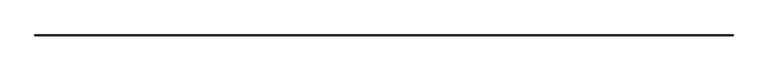
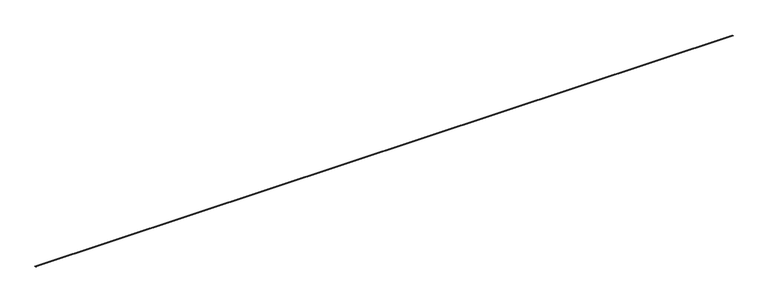
"""IFC4 building model written with IfcOpenShell, lengths in millimetres: proxy geometry, Generic Models 7:Generic Models 1:6:Generic Models 1:6 : Generic Models 7:Generic Models 1:337419:20 : Generic Models 7:Generic Models 1:6:Generic Models 1:6 : Generic Models 7:Generic Models 1:337419:312901."""

from ifc_helpers import new_model, si_unit, frame, origin, place, context, project, spatial, polyline, outline, extrude, source, transform, mapped, element, save


def generic_models_84a8ac5e(model_context):
    return source(origin(), model_context, "Body", "SweptSolid", [
        extrude(outline(polyline([(-579024.8509681, 4.5309106), (-579024.8509681, 24.3756332), (-579021.6759681, 24.3756332), (-579021.6759681, 7.7059106), (-578858.9280519, 7.7059106), (-578858.9280519, 4.5309106), (-579024.8509681, 4.5309106)])), frame((557771.6867239, 0.0, 0.0), z_axis=(1.0, 0.0, 0.0), x_axis=(0.0, 1.0, 0.0)), (0.0, 0.0, 1.0), 109559.725),
    ])


if __name__ == "__main__":
    model = new_model("IFC4")
    model_context = context("Model", 3, world=origin())
    ifc_project = project(units=[si_unit("LENGTHUNIT", "METRE", prefix="MILLI")], contexts=[model_context])
    site = spatial("IfcSite", under=ifc_project)
    building = spatial("IfcBuilding", under=site)
    placement = place(None, origin())
    generic_models_shape = generic_models_84a8ac5e(model_context)
    element("IfcBuildingElementProxy", 1, Name="Generic Models 7:Generic Models 1:6:Generic Models 1:6 : Generic Models 7:Generic Models 1:337419:20 : Generic Models 7:Generic Models 1:6:Generic Models 1:6 : Generic Models 7:Generic Models 1:337419:312901", ObjectType="Generic Models 7:Generic Models 1:6:Generic Models 1:6 : Generic Models 7:Generic Models 1:337419:20 : Generic Models 7:Generic Models 1:6:Generic Models 1:6 : Generic Models 7:Generic Models 1:337419:312901", at=placement, inside=building, context=model_context, shape_type="MappedRepresentation", body=[
        mapped(generic_models_shape, transform((0.0, 0.0, 0.0), x_axis=(1.0, 0.0, 0.0), y_axis=(0.0, 1.0, 0.0), z_axis=(0.0, 0.0, 1.0))),
    ])
    save(model, "model.ifc")

# Revit data of these elements
# Type "Generic Models 7:Generic Models 1:6:Generic Models 1:6 : Generic Models 7:Generic Models 1:337419:20 : Generic Models 7:Generic Models 1:6:Generic Models 1:6 : Generic Models 7:Generic Models 1:337419:312901"
#   NameOverride = "Generic Models 7:Generic Models 1:6:Generic Models 1:6 : Generic Models 7:Generic Models 1:337419:312901"
#   ObjectTypeOverride = "Generic Models 1:6 : Generic Models 7:Generic Models 1:337419"
#   Reference = "Generic Models 1"
#   Tag = "312901"
# Element 1 (IfcBuildingElementProxy, "Generic Models 7:Generic Models 1:6:Generic Models 1:6 : Generic Models 7:Generic Models 1:337419:20 : Generic Models 7:Generic Models 1:6:Generic Models 1:6 : Generic Models 7:Generic Models 1:337419:312901")
#   Materials on its faces: "STAINLESS STEEL BENT PLATE (FLASHING)"
# Materials
#   "STAINLESS STEEL BENT PLATE (FLASHING)": class "Unassigned", colour RGB 210 209 208, transparency 0, Cost = 0
